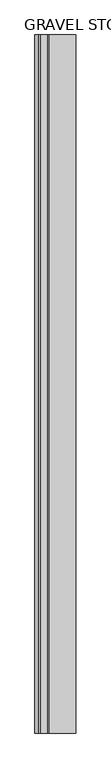
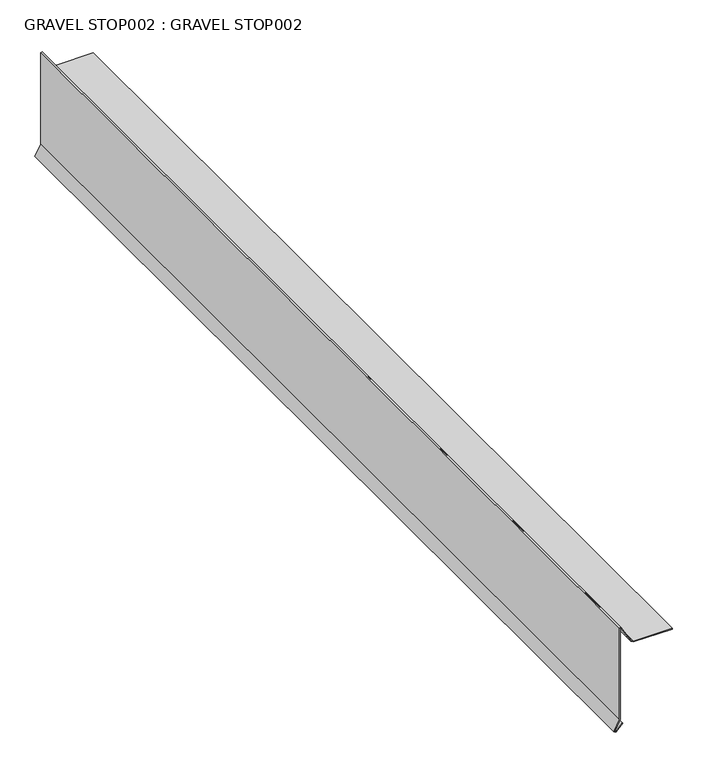
"""IFC4 building model written with IfcOpenShell, lengths in millimetres: proxy geometry, GRAVEL STOP002 : GRAVEL STOP002."""

from ifc_helpers import new_model, si_unit, frame, origin, place, context, project, spatial, polyline, outline, extrude, source, transform, mapped, element, save


def gravel_stop002_gravel_stop002_e62ea456(model_context):
    return source(origin(), model_context, "Body", "SweptSolid", [
        extrude(outline(polyline([(40077.410403, -5045.5157154), (40091.8049, -5031.1212184), (40092.8027062, -5032.1190245), (40079.2807815, -5045.6409492), (40080.9054201, -5047.7705993), (40101.495749, -5036.5295796), (40293.447969, -5036.5295796), (40293.699878, -5035.5894424), (40258.5078708, -5015.2713276), (40255.9633674, -5010.8641185), (40255.9633674, -4933.0281058), (40257.3744784, -4933.0281058), (40257.3744784, -5010.4860124), (40259.5408757, -5014.2383227), (40295.3431515, -5034.9087762), (40294.5307525, -5037.9406906), (40101.8558531, -5037.9406906), (40080.5182783, -5049.5896595), (40077.410403, -5045.5157154)])), frame((0.0, -1052.8906573, 0.0), z_axis=(0.0, 1.0, 0.0), x_axis=(0.0, 0.0, 1.0)), (0.0, 0.0, 1.0), 2000.25),
    ])


if __name__ == "__main__":
    model = new_model("IFC4")
    model_context = context("Model", 3, world=origin())
    ifc_project = project(units=[si_unit("LENGTHUNIT", "METRE", prefix="MILLI")], contexts=[model_context])
    site = spatial("IfcSite", under=ifc_project)
    building = spatial("IfcBuilding", under=site)
    placement = place(None, origin())
    gravel_stop002_gravel_stop002_shape = gravel_stop002_gravel_stop002_e62ea456(model_context)
    element("IfcBuildingElementProxy", 1, Name="GRAVEL STOP002 : GRAVEL STOP002", ObjectType="GRAVEL STOP002 : GRAVEL STOP002", at=placement, inside=building, context=model_context, shape_type="MappedRepresentation", body=[
        mapped(gravel_stop002_gravel_stop002_shape, transform((0.0, 0.0, 0.0), x_axis=(1.0, 0.0, 0.0), y_axis=(0.0, 1.0, 0.0), z_axis=(0.0, 0.0, 1.0))),
    ])
    save(model, "model.ifc")

# Revit data of these elements
# Type "GRAVEL STOP002 : GRAVEL STOP002"
#   NameOverride = "GRAVEL STOP002"
# Element 1 (IfcBuildingElementProxy, "GRAVEL STOP002 : GRAVEL STOP002")
#   Materials on its faces: "GRAVEL STOP REQUIRED WITH GRAVEL SURFACE SYSTEMS"
# Materials
#   "GRAVEL STOP REQUIRED WITH GRAVEL SURFACE SYSTEMS": class "Unassigned", colour RGB 170 170 127, transparency 0
